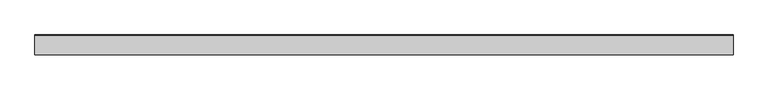
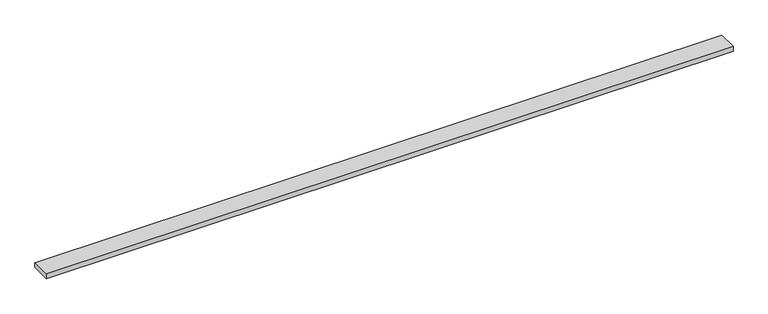
"""IFC4 building model written with IfcOpenShell, lengths in millimetres: proxy geometry, Generic Models 7:Generic Models 1:2:Generic Models 1:2 : Generic Models 7:Generic Models 1:337419:1 : Generic Models 7:Generic Models 1:2:Generic Models 1:2 : Generic Models 7:Generic Models 1:337419:306751."""

import ifcopenshell
import ifcopenshell.guid

model = None  # the IFC model being written
_history = None  # IfcOwnerHistory: only IFC2X3 demands one
_inside = {}  # id of a spatial element -> (the spatial element, [elements in it])
_under = {}  # id of a project, library or spatial element -> (it, [spatial elements below it])
_declared = {}  # id of a project -> (the project, [libraries it declares])
_typed = {}  # id of a type object -> (the type object, [elements of that type])
_made_of = {}  # id of a material, layer set ... -> (it, [elements and type objects made of it])


def new_model(schema):
    """Start an empty IFC model of exactly this schema.

    Asked for "IFC4X3", IfcOpenShell would pick the latest addendum, in which some entities
    have other attributes; the version numbers below select the first issue.
    IFC2X3 requires an IfcOwnerHistory on every rooted entity: one is made here for all.
    """
    global model, _history
    if schema == "IFC4X3":
        model = ifcopenshell.file(schema_version=(4, 3, 0, 0))
    else:
        model = ifcopenshell.file(schema=schema)
    _inside.clear()
    _under.clear()
    _declared.clear()
    _typed.clear()
    _made_of.clear()
    _history = None
    if model.schema == "IFC2X3":
        org = make("IfcOrganization", Name="unknown")
        user = make(
            "IfcPersonAndOrganization",
            ThePerson=make("IfcPerson", FamilyName="unknown"),
            TheOrganization=org,
        )
        app = make(
            "IfcApplication",
            ApplicationDeveloper=org,
            Version="unknown",
            ApplicationFullName="unknown",
            ApplicationIdentifier="unknown",
        )
        _history = make(
            "IfcOwnerHistory",
            OwningUser=user,
            OwningApplication=app,
            ChangeAction="ADDED",
            CreationDate=0,
        )
    return model


def make(cls, **values):
    """One entity of the class cls with the attributes given. An attribute that is None is left unset."""
    return model.create_entity(
        cls, **{name: value for name, value in values.items() if value is not None}
    )


def rooted(cls, **values):
    """An entity with a GlobalId (a new one), such as an element, a storey or a relation."""
    return make(cls, GlobalId=ifcopenshell.guid.new(), OwnerHistory=_history, **values)


def si_unit(unit_type, name, prefix=None):
    """IfcSIUnit, for example si_unit("LENGTHUNIT", "METRE", prefix="MILLI")."""
    return make("IfcSIUnit", UnitType=unit_type, Prefix=prefix, Name=name)


def assignment(units):
    """IfcUnitAssignment: the units of a project."""
    return None if units is None else make("IfcUnitAssignment", Units=units)


def point(xyz):
    """IfcCartesianPoint."""
    return None if xyz is None else make("IfcCartesianPoint", Coordinates=xyz)


def direction(xyz):
    """IfcDirection."""
    return None if xyz is None else make("IfcDirection", DirectionRatios=xyz)


def frame(location, z_axis=None, x_axis=None):
    """IfcAxis2Placement3D, a coordinate frame: its origin and axes. An axis left out is left unset."""
    return make(
        "IfcAxis2Placement3D",
        Location=point(location),
        Axis=direction(z_axis),
        RefDirection=direction(x_axis),
    )


def origin():
    """The frame at (0, 0, 0) with its axes left unset."""
    return frame((0.0, 0.0, 0.0))


def place(relative_to, where):
    """IfcLocalPlacement: puts the frame where relative to a parent placement (None: the world)."""
    return make(
        "IfcLocalPlacement", PlacementRelTo=relative_to, RelativePlacement=where
    )


def context(
    kind, dimensions, precision=None, world=None, true_north=None, identifier=None
):
    """IfcGeometricRepresentationContext, for example the 3D "Model" context."""
    return make(
        "IfcGeometricRepresentationContext",
        ContextIdentifier=identifier,
        ContextType=kind,
        CoordinateSpaceDimension=dimensions,
        Precision=precision,
        WorldCoordinateSystem=world,
        TrueNorth=true_north,
    )


def project(units=None, contexts=None):
    """IfcProject with its units and contexts."""
    return rooted(
        "IfcProject",
        Name="project",
        RepresentationContexts=contexts,
        UnitsInContext=assignment(units),
    )


def spatial(cls, under=None, at=None, **own):
    """A site, building, storey or space (cls), placed at a placement, below another one or the project."""
    s = rooted(cls, ObjectPlacement=at, **own)
    if under is not None:
        _under.setdefault(under.id(), (under, []))[1].append(s)
    return s


def polyline(points):
    """IfcPolyline through the points."""
    return make("IfcPolyline", Points=[point(p) for p in points])


def outline(outer, holes=None, kind="AREA"):
    """IfcArbitraryClosedProfileDef: a profile drawn as a closed curve; with holes, ...WithVoids."""
    if holes is None:
        return make("IfcArbitraryClosedProfileDef", ProfileType=kind, OuterCurve=outer)
    return make(
        "IfcArbitraryProfileDefWithVoids",
        ProfileType=kind,
        OuterCurve=outer,
        InnerCurves=holes,
    )


def extrude(swept, where, along, depth):
    """IfcExtrudedAreaSolid: the profile swept, set in the frame where, extruded along a direction by depth."""
    return make(
        "IfcExtrudedAreaSolid",
        SweptArea=swept,
        Position=where,
        ExtrudedDirection=direction(along),
        Depth=depth,
    )


def shape(context_of_items, identifier, shape_type, items):
    """IfcShapeRepresentation: the items that make up one representation, for example the "Body"."""
    return make(
        "IfcShapeRepresentation",
        ContextOfItems=context_of_items,
        RepresentationIdentifier=identifier,
        RepresentationType=shape_type,
        Items=items,
    )


def source(mapping_origin, context_of_items, identifier, shape_type, items):
    """IfcRepresentationMap: a shape defined once, which mapped items show again and again."""
    return make(
        "IfcRepresentationMap",
        MappingOrigin=mapping_origin,
        MappedRepresentation=shape(context_of_items, identifier, shape_type, items),
    )


def transform(
    local_origin,
    x_axis=None,
    y_axis=None,
    z_axis=None,
    scale=None,
    scale2=None,
    scale3=None,
    uniform=True,
):
    """IfcCartesianTransformationOperator3D, or its non-uniform kind. x_axis, y_axis, z_axis: its Axis1, 2, 3."""
    if uniform:
        return make(
            "IfcCartesianTransformationOperator3D",
            Axis1=direction(x_axis),
            Axis2=direction(y_axis),
            LocalOrigin=point(local_origin),
            Scale=scale,
            Axis3=direction(z_axis),
        )
    return make(
        "IfcCartesianTransformationOperator3DnonUniform",
        Axis1=direction(x_axis),
        Axis2=direction(y_axis),
        LocalOrigin=point(local_origin),
        Scale=scale,
        Axis3=direction(z_axis),
        Scale2=scale2,
        Scale3=scale3,
    )


def mapped(mapping_source, mapping_target):
    """IfcMappedItem: shows the shape of a source again, moved by a transform."""
    return make(
        "IfcMappedItem", MappingSource=mapping_source, MappingTarget=mapping_target
    )


def made_of(thing, what):
    """Note that an element or type object is made of a material, layer set ...; save() writes the relation."""
    if what is not None:
        _made_of.setdefault(what.id(), (what, []))[1].append(thing)
    return thing


def element(
    cls,
    number,
    at=None,
    inside=None,
    cuts=None,
    type_object=None,
    material=None,
    context=None,
    identifier="Body",
    shape_type=None,
    held_by="IfcProductDefinitionShape",
    body=None,
    shapes=None,
    **own,
):
    """One element of the class cls, such as IfcWall. Its Tag is "e" and its number.

    at: its placement. inside: the storey or other place that contains it. cuts: it is an
    opening in that element (IfcRelVoidsElement). A single representation is given by context,
    identifier, shape_type and body (its items); several are given by shapes. held_by: the class
    of the entity that holds the representations. save() writes the other relations.
    """
    e = rooted(cls, Tag="e%d" % number, ObjectPlacement=at, **own)
    if body is not None:
        shapes = [shape(context, identifier, shape_type, body)]
    if shapes is not None:
        e.Representation = make(held_by, Representations=shapes)
    if inside is not None:
        _inside.setdefault(inside.id(), (inside, []))[1].append(e)
    if cuts is not None:
        rooted(
            "IfcRelVoidsElement", RelatingBuildingElement=cuts, RelatedOpeningElement=e
        )
    if type_object is not None:
        _typed.setdefault(type_object.id(), (type_object, []))[1].append(e)
    return made_of(e, material)


def aggregate(whole, parts):
    """IfcRelAggregates: a whole, such as a stair, and the parts it consists of."""
    return rooted("IfcRelAggregates", RelatingObject=whole, RelatedObjects=parts)


def save(model, path):
    """Write the relations noted so far, then the file.

    IfcRelAggregates (storeys below a building ...), IfcRelContainedInSpatialStructure (elements
    in a storey), IfcRelDefinesByType, IfcRelAssociatesMaterial and IfcRelDeclares: one each for
    every whole, place, type object, material and project.
    """
    for whole, parts in _under.values():
        aggregate(whole, parts)
    for where, things in _inside.values():
        rooted(
            "IfcRelContainedInSpatialStructure",
            RelatedElements=things,
            RelatingStructure=where,
        )
    for kind, things in _typed.values():
        rooted("IfcRelDefinesByType", RelatedObjects=things, RelatingType=kind)
    for what, things in _made_of.values():
        rooted("IfcRelAssociatesMaterial", RelatedObjects=things, RelatingMaterial=what)
    for by, libraries in _declared.values():
        rooted("IfcRelDeclares", RelatingContext=by, RelatedDefinitions=libraries)
    model.write(path)


def generic_models_fccb1870(model_context):
    return source(origin(), model_context, "Body", "SweptSolid", [
        extrude(outline(polyline([(-567923.3188012, 8546.1818773), (-567923.3188012, 8584.2818773), (-567786.1940035, 8584.2818773), (-567783.6188012, 8581.706675), (-567783.6188012, 8546.1818773), (-567923.3188012, 8546.1818773)])), frame((591306.0367242, 0.0, 0.0), z_axis=(1.0, 0.0, 0.0), x_axis=(0.0, 1.0, 0.0)), (0.0, 0.0, 1.0), 4876.8),
    ])


if __name__ == "__main__":
    model = new_model("IFC4")
    model_context = context("Model", 3, world=origin())
    ifc_project = project(units=[si_unit("LENGTHUNIT", "METRE", prefix="MILLI")], contexts=[model_context])
    site = spatial("IfcSite", under=ifc_project)
    building = spatial("IfcBuilding", under=site)
    placement = place(None, origin())
    generic_models_shape = generic_models_fccb1870(model_context)
    element("IfcBuildingElementProxy", 1, Name="Generic Models 7:Generic Models 1:2:Generic Models 1:2 : Generic Models 7:Generic Models 1:337419:1 : Generic Models 7:Generic Models 1:2:Generic Models 1:2 : Generic Models 7:Generic Models 1:337419:306751", ObjectType="Generic Models 7:Generic Models 1:2:Generic Models 1:2 : Generic Models 7:Generic Models 1:337419:1 : Generic Models 7:Generic Models 1:2:Generic Models 1:2 : Generic Models 7:Generic Models 1:337419:306751", at=placement, inside=building, context=model_context, shape_type="MappedRepresentation", body=[
        mapped(generic_models_shape, transform((0.0, 0.0, 0.0), x_axis=(1.0, 0.0, 0.0), y_axis=(0.0, 1.0, 0.0), z_axis=(0.0, 0.0, 1.0))),
    ])
    save(model, "model.ifc")

# Revit data of these elements
# Type "Generic Models 7:Generic Models 1:2:Generic Models 1:2 : Generic Models 7:Generic Models 1:337419:1 : Generic Models 7:Generic Models 1:2:Generic Models 1:2 : Generic Models 7:Generic Models 1:337419:306751"
#   NameOverride = "Generic Models 7:Generic Models 1:2:Generic Models 1:2 : Generic Models 7:Generic Models 1:337419:306751"
#   ObjectTypeOverride = "Generic Models 1:2 : Generic Models 7:Generic Models 1:337419"
#   Reference = "Generic Models 1"
#   Tag = "306751"
# Element 1 (IfcBuildingElementProxy, "Generic Models 7:Generic Models 1:2:Generic Models 1:2 : Generic Models 7:Generic Models 1:337419:1 : Generic Models 7:Generic Models 1:2:Generic Models 1:2 : Generic Models 7:Generic Models 1:337419:306751")
#   Materials on its faces: "FIRE RETARDTANT WOOD BLOCKING - SIZE AS NECESSARY"
# Materials
#   "FIRE RETARDTANT WOOD BLOCKING - SIZE AS NECESSARY": class "Wood", colour RGB 144 113 62, transparency 0, Description = "Pinus Echinata", Cost = 0
